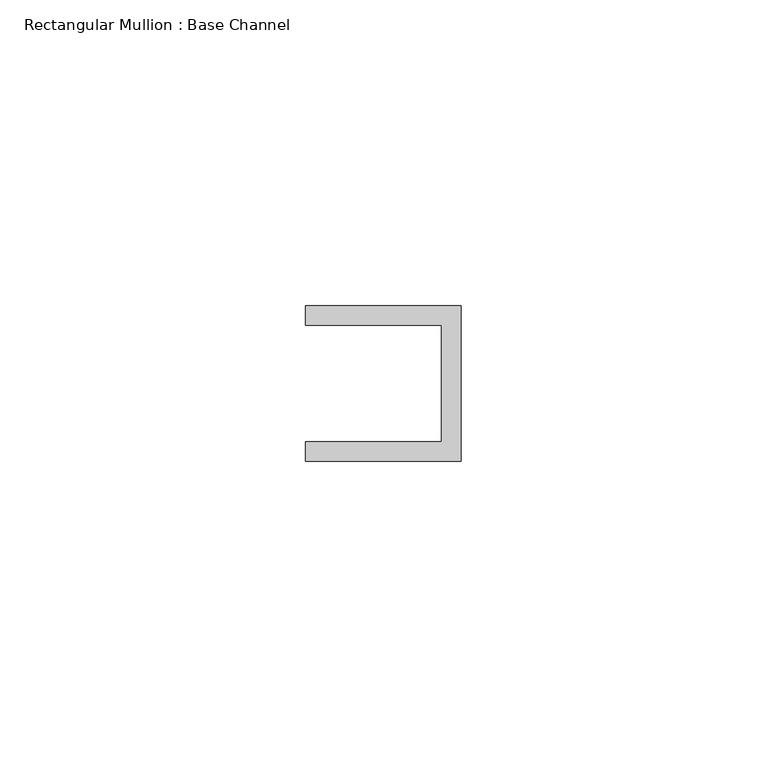
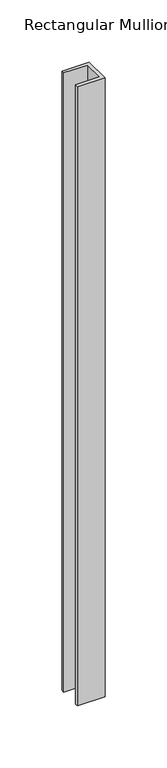
"""IFC4 building model written with IfcOpenShell, lengths in millimetres: member geometry, Rectangular Mullion : Base Channel."""

from ifc_helpers import new_model, si_unit, frame, origin, place, context, project, spatial, polyline, outline, extrude, source, transform, mapped, element, save


def rectangular_mullion_base_channel_22be779d(model_context):
    return source(origin(), model_context, "Body", "SweptSolid", [
        extrude(outline(polyline([(0.0, -12.7), (-25.4, -12.7), (-25.4, -9.525), (-3.175, -9.525), (-3.175, 9.525), (-25.4, 9.525), (-25.4, 12.7), (0.0, 12.7), (0.0, -12.7)])), frame((0.0, 0.0, -609.6), z_axis=(0.0, 0.0, 1.0), x_axis=(1.0, 0.0, 0.0)), (0.0, 0.0, 1.0), 609.6),
    ])


if __name__ == "__main__":
    model = new_model("IFC4")
    model_context = context("Model", 3, world=origin())
    ifc_project = project(units=[si_unit("LENGTHUNIT", "METRE", prefix="MILLI")], contexts=[model_context])
    site = spatial("IfcSite", under=ifc_project)
    building = spatial("IfcBuilding", under=site)
    placement = place(None, origin())
    rectangular_mullion_base_channel_shape = rectangular_mullion_base_channel_22be779d(model_context)
    element("IfcMember", 1, ObjectType="Rectangular Mullion : Base Channel", at=placement, inside=building, context=model_context, shape_type="MappedRepresentation", body=[
        mapped(rectangular_mullion_base_channel_shape, transform((0.0, 0.0, 0.0), x_axis=(1.0, 0.0, 0.0), y_axis=(0.0, 1.0, 0.0), z_axis=(0.0, 0.0, 1.0))),
    ])
    save(model, "model.ifc")

# Revit data of these elements
# Type "Rectangular Mullion : Base Channel"
#   built-in parameter 1007322 = 0.0833333 (stored number, unit not read)
#   built-in parameter 1007321 = 0.0416667 (stored number, unit not read)
#   built-in parameter 1007320 = -0.03125 (stored number, unit not read)
# Element 1 (IfcMember, "Rectangular Mullion : Base Channel")
#   Materials on its faces: "ALUM"
# Materials
#   "ALUM": class "Generic", colour RGB 157 157 157, transparency 0, Cost = 0
